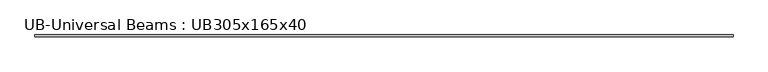
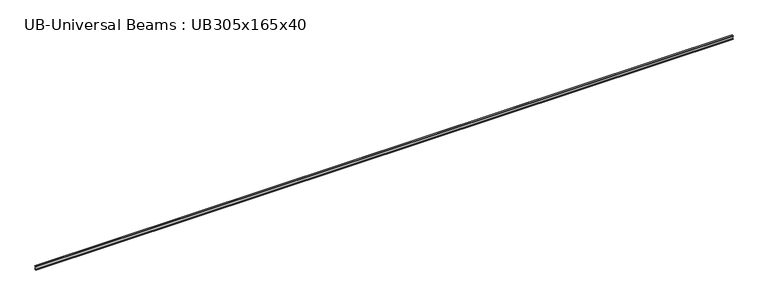
"""IFC4 building model written with IfcOpenShell, lengths in millimetres: beam geometry, UB-Universal Beams : UB305x165x40."""

from ifc_helpers import new_model, si_unit, point, frame, frame_2d, origin, place, context, project, spatial, polyline, circle_curve, trimmed, segment, composite_curve, outline, extrude, source, transform, mapped, element, save


def ub_universal_beams_ub305x165x40_9b6b5504(model_context):
    return source(origin(), model_context, "Body", "SweptSolid", [
        extrude(outline(composite_curve([segment(polyline([(82.5, -141.5), (82.5, -151.7), (-82.5, -151.7), (-82.5, -141.5), (-11.9, -141.5)]), True, "CONTINUOUS"), segment(trimmed(circle_curve(frame_2d((-11.9, -132.6)), 8.9), [point((-11.9, -141.5))], [point((-3.0, -132.6))], True, "CARTESIAN"), True, "CONTINUOUS"), segment(polyline([(-3.0, -132.6), (-3.0, 132.6)]), True, "CONTINUOUS"), segment(trimmed(circle_curve(frame_2d((-11.9, 132.6)), 8.9), [point((-3.0, 132.6))], [point((-11.9, 141.5))], True, "CARTESIAN"), True, "CONTINUOUS"), segment(polyline([(-11.9, 141.5), (-82.5, 141.5), (-82.5, 151.7), (82.5, 151.7), (82.5, 141.5), (11.9, 141.5)]), True, "CONTINUOUS"), segment(trimmed(circle_curve(frame_2d((11.9, 132.6)), 8.9), [point((11.9, 141.5))], [point((3.0, 132.6))], True, "CARTESIAN"), True, "CONTINUOUS"), segment(polyline([(3.0, 132.6), (3.0, -132.6)]), True, "CONTINUOUS"), segment(trimmed(circle_curve(frame_2d((11.9, -132.6)), 8.9), [point((3.0, -132.6))], [point((11.9, -141.5))], True, "CARTESIAN"), True, "CONTINUOUS"), segment(polyline([(11.9, -141.5), (82.5, -141.5)]), True, "CONTINUOUS")], self_intersect=False)), frame((-30962.3, 0.0, 0.0), z_axis=(1.0, 0.0, 0.0), x_axis=(0.0, 1.0, 0.0)), (0.0, 0.0, 1.0), 61924.6),
    ])


if __name__ == "__main__":
    model = new_model("IFC4")
    model_context = context("Model", 3, world=origin())
    ifc_project = project(units=[si_unit("LENGTHUNIT", "METRE", prefix="MILLI")], contexts=[model_context])
    site = spatial("IfcSite", under=ifc_project)
    building = spatial("IfcBuilding", under=site)
    placement = place(None, origin())
    ub_universal_beams_ub305x165x40_shape = ub_universal_beams_ub305x165x40_9b6b5504(model_context)
    element("IfcBeam", 1, ObjectType="UB-Universal Beams : UB305x165x40", at=placement, inside=building, context=model_context, shape_type="MappedRepresentation", body=[
        mapped(ub_universal_beams_ub305x165x40_shape, transform((0.0, 0.0, 0.0), x_axis=(1.0, 0.0, 0.0), y_axis=(0.0, 1.0, 0.0), z_axis=(0.0, 0.0, 1.0))),
    ])
    save(model, "model.ifc")

# Revit data of these elements
# Type "UB-Universal Beams : UB305x165x40"
#   Section Name Key = "UB305X165X40"
#   Width = 16.5 cm
#   Web Thickness = 0.6 cm
#   Web Fillet = 0.89 cm
#   Warping Constant = 164000.0 cm⁶
#   Torsional Moment of Inertia = 14.70 cm⁴
#   Section Area = 51.3 cm²
#   Plastic Modulus weak axis = 142.0 cm³
#   Plastic Modulus strong axis = 623.0 cm³
#   Nominal Weight = 40.2999 kgf/m
#   Moment of Inertia weak axis = 764.00 cm⁴
#   Moment of Inertia strong axis = 8503.00 cm⁴
#   Height = 30.34 cm
#   Flange Thickness = 1.02 cm
#   Elastic Modulus weak axis = 92.6 cm³
#   Elastic Modulus strong axis = 560.0 cm³
#   Centroid Vertical = 15.17 cm
#   Centroid Horizontal = 8.25 cm
#   Bolt Spacing = 9.0 cm
#   Length [instance default] = 1500 mm
#   Structural Material [instance default] = Metal - Steel 43-275
#   Type Comments = ""
#   Assembly Code = ""
# Element 1 (IfcBeam, "UB-Universal Beams : UB305x165x40")
#   Materials on its faces: "Metal - Steel 43-275"
# Materials
#   "Metal - Steel 43-275": class "Metal", colour RGB 247 247 247, transparency 0, Cost = 0
